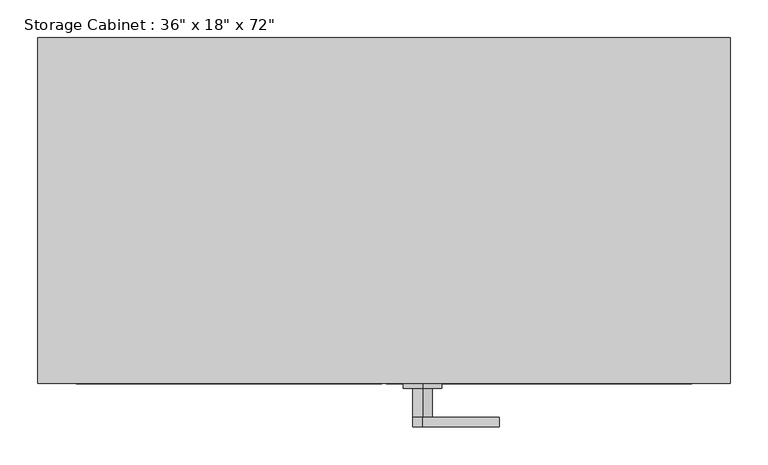
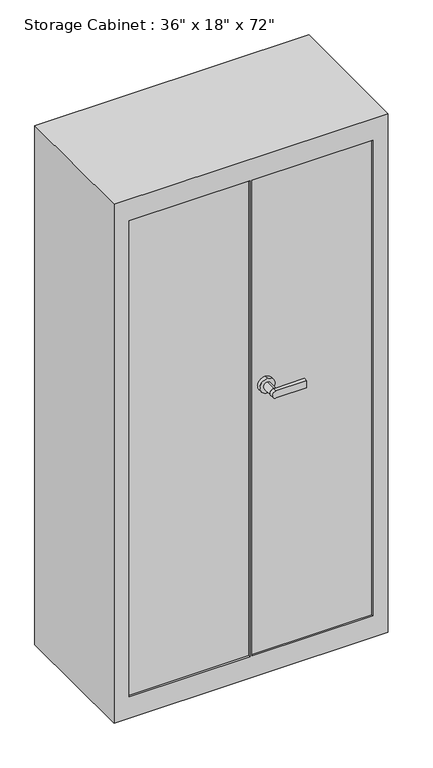
"""IFC4 building model written with IfcOpenShell, lengths in millimetres: furniture geometry."""

from ifc_helpers import new_model, si_unit, point, frame, frame_2d, origin, place, context, project, spatial, polyline, circle_curve, trimmed, segment, composite_curve, outline, extrude, faceted_brep, source, transform, mapped, element, save


def furniture_a97b73e9(model_context):
    return source(origin(), model_context, "Body", "SolidModel", [
        extrude(outline(composite_curve([segment(polyline([(1028.7, 152.5427411), (1028.7, 50.9427411)]), True, "CONTINUOUS"), segment(trimmed(circle_curve(frame_2d((1016.0, 50.9427411)), 12.7), [point((1028.7, 50.9427411))], [point((1003.3, 50.9427411))], False, "CARTESIAN"), True, "CONTINUOUS"), segment(polyline([(1003.3, 50.9427411), (1003.3, 152.5427411), (1028.7, 152.5427411)]), True, "CONTINUOUS")], self_intersect=False)), frame((0.0, -285.75, 0.0), z_axis=(0.0, 1.0, 0.0), x_axis=(0.0, 0.0, 1.0)), (0.0, 0.0, 1.0), 12.7),
        extrude(outline(composite_curve([segment(trimmed(circle_curve(frame_2d((1016.0, 50.9427411)), 12.7), [point((1028.7, 50.9427411))], [point((1003.3, 50.9427411))], False, "CARTESIAN"), True, "CONTINUOUS"), segment(trimmed(circle_curve(frame_2d((1016.0, 50.9427411)), 12.7), [point((1003.3, 50.9427411))], [point((1028.7, 50.9427411))], False, "CARTESIAN"), True, "CONTINUOUS")], self_intersect=False)), frame((0.0, -273.05, 0.0), z_axis=(0.0, 1.0, 0.0), x_axis=(0.0, 0.0, 1.0)), (0.0, 0.0, 1.0), 38.1),
        extrude(outline(composite_curve([segment(trimmed(circle_curve(frame_2d((1016.0, 50.9427411)), 25.4), [point((1041.4, 50.9427411))], [point((990.6, 50.9427411))], False, "CARTESIAN"), True, "CONTINUOUS"), segment(trimmed(circle_curve(frame_2d((1016.0, 50.9427411)), 25.4), [point((990.6, 50.9427411))], [point((1041.4, 50.9427411))], False, "CARTESIAN"), True, "CONTINUOUS")], self_intersect=False)), frame((0.0, -234.95, 0.0), z_axis=(0.0, 1.0, 0.0), x_axis=(0.0, 0.0, 1.0)), (0.0, 0.0, 1.0), 12.7),
        faceted_brep([(457.2, -228.6, 1828.8), (457.2, 228.6, 1828.8), (-457.2, 228.6, 1828.8), (-457.2, -228.6, 1828.8), (457.2, -228.6, 0.0), (-457.2, -228.6, 0.0), (-457.2, 228.6, 0.0), (457.2, 228.6, 0.0), (406.4, -228.6, 1752.6), (406.4, -228.6, 76.2), (3.175, -228.6, 76.2), (3.175, -228.6, 1752.6), (-406.4, -228.6, 1752.6), (-3.175, -228.6, 1752.6), (-3.175, -228.6, 76.2), (-406.4, -228.6, 76.2), (406.4, -222.25, 76.2), (406.4, -222.25, 1752.6), (3.175, -222.25, 1752.6), (3.175, -222.25, 76.2), (-3.175, -222.25, 1752.6), (-406.4, -222.25, 1752.6), (-406.4, -222.25, 76.2), (-3.175, -222.25, 76.2)], [[[0, 1, 2, 3]], [[4, 5, 6, 7]], [[1, 0, 4, 7]], [[2, 1, 7, 6]], [[3, 2, 6, 5]], [[0, 3, 5, 4], [8, 9, 10, 11], [12, 13, 14, 15]], [[16, 17, 18, 19]], [[17, 16, 9, 8]], [[18, 17, 8, 11]], [[19, 18, 11, 10]], [[16, 19, 10, 9]], [[20, 21, 22, 23]], [[21, 20, 13, 12]], [[22, 21, 12, 15]], [[23, 22, 15, 14]], [[20, 23, 14, 13]]]),
    ])


if __name__ == "__main__":
    model = new_model("IFC4")
    model_context = context("Model", 3, world=origin())
    ifc_project = project(units=[si_unit("LENGTHUNIT", "METRE", prefix="MILLI")], contexts=[model_context])
    site = spatial("IfcSite", under=ifc_project)
    building = spatial("IfcBuilding", under=site)
    placement = place(None, origin())
    furniture_shape = furniture_a97b73e9(model_context)
    element("IfcFurniture", 1, ObjectType="Storage Cabinet : 36\" x 18\" x 72\"", at=placement, inside=building, context=model_context, shape_type="MappedRepresentation", body=[
        mapped(furniture_shape, transform((0.0, 0.0, 0.0), x_axis=(1.0, 0.0, 0.0), y_axis=(0.0, 1.0, 0.0), z_axis=(0.0, 0.0, 1.0))),
    ])
    save(model, "model.ifc")

# Revit data of these elements
# Type "Storage Cabinet : 36\" x 18\" x 72\""
#   Depth = 1' - 6"
#   Height = 6' - 0"
#   Width = 3' - 0"
#   Default Elevation = 0
# Element 1 (IfcFurniture, "Storage Cabinet : 36\" x 18\" x 72\"")
#   Materials on its faces: "Chrome"
# Materials
#   "Chrome": class "Unassigned", colour RGB 222 227 228, transparency 0
